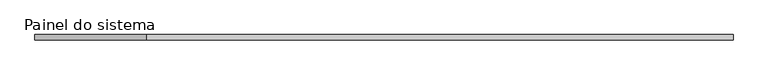
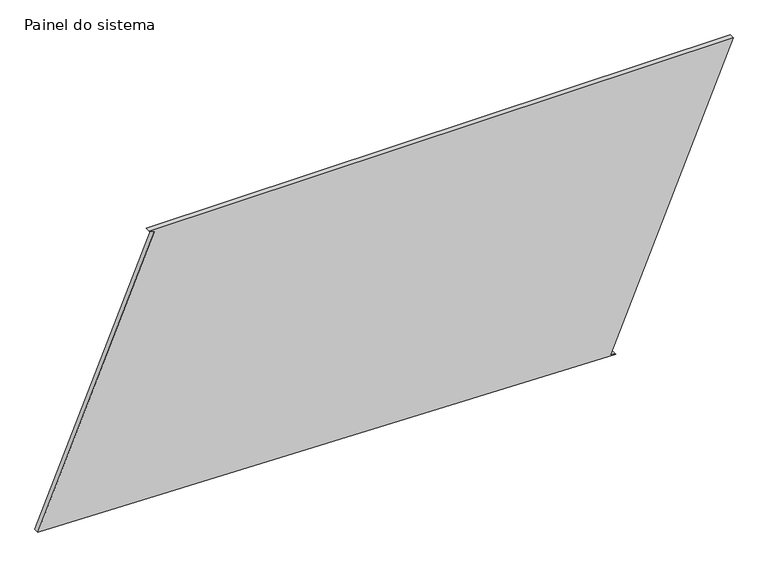
"""IFC4 building model written with IfcOpenShell, lengths in millimetres: plate geometry, Painel do sistema : Envidraçado."""

from ifc_helpers import new_model, si_unit, frame, origin, place, context, project, spatial, polyline, outline, extrude, source, transform, mapped, element, save


def painel_do_sistema_0da5ea92(model_context):
    return source(origin(), model_context, "Body", "SweptSolid", [
        extrude(outline(polyline([(0.0, 1089.3180675), (9.6723918, 1066.2649801), (1388.9907842, 1644.9860717), (1388.9907842, -1117.7989053), (1379.3183925, -1094.7458179), (67.8809602, -1644.9860717), (0.0, 1089.3180675)])), frame((0.0, 24.5, 0.0), z_axis=(0.0, 1.0, 0.0), x_axis=(0.0, 0.0, 1.0)), (0.0, 0.0, 1.0), 25.0),
    ])


if __name__ == "__main__":
    model = new_model("IFC4")
    model_context = context("Model", 3, world=origin())
    ifc_project = project(units=[si_unit("LENGTHUNIT", "METRE", prefix="MILLI")], contexts=[model_context])
    site = spatial("IfcSite", under=ifc_project)
    building = spatial("IfcBuilding", under=site)
    placement = place(None, origin())
    painel_do_sistema_shape = painel_do_sistema_0da5ea92(model_context)
    element("IfcPlate", 1, ObjectType="Painel do sistema : Envidraçado", at=placement, inside=building, context=model_context, shape_type="MappedRepresentation", body=[
        mapped(painel_do_sistema_shape, transform((0.0, 0.0, 0.0), x_axis=(1.0, 0.0, 0.0), y_axis=(0.0, 1.0, 0.0), z_axis=(0.0, 0.0, 1.0))),
    ])
    save(model, "model.ifc")

# Revit data of these elements
# Type "Painel do sistema : Envidraçado"
#   Construction Type Id = "GSP4R"
#   Analytic Construction = "Vidraça única Pilkington 1/8 pol"
#   Visual Light Transmittance = 0.9
#   Solar Heat Gain Coefficient = 0.86
#   Heat Transfer Coefficient (U) = 6.7069 W/(m²·K)
# Element 1 (IfcPlate, "Painel do sistema : Envidraçado")
#   Materials on its faces: "Vidro"
# Materials
#   "Vidro": class "Vidro", colour RGB 0 128 192, transparency 0.9, Description = "Vidro de sílica", Cost = 0
